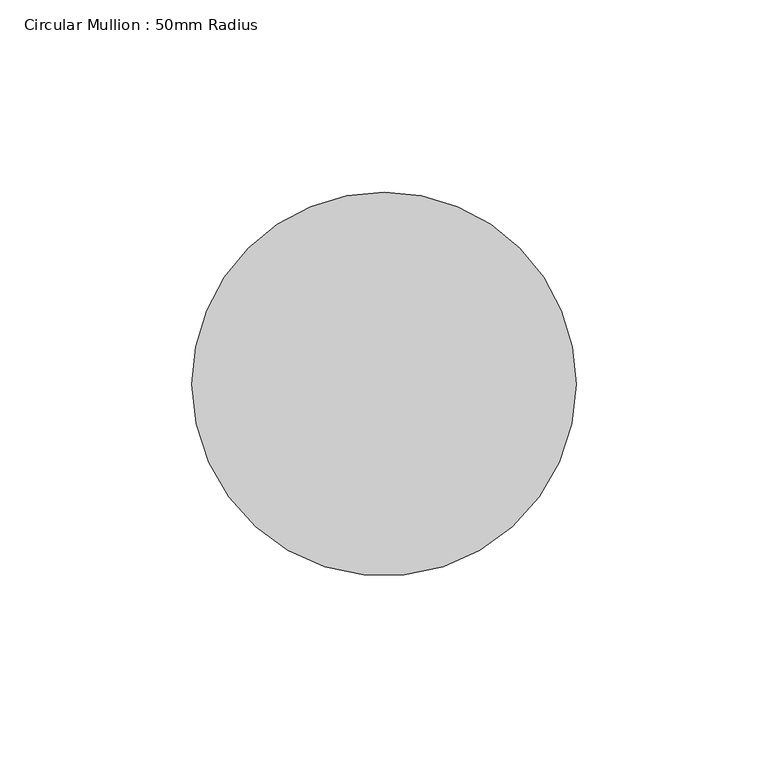
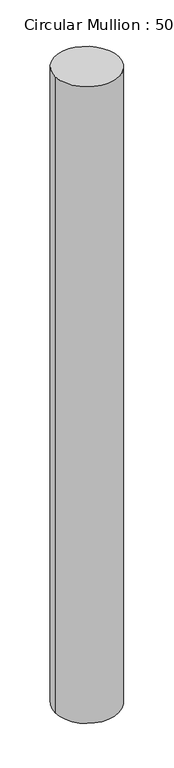
"""IFC4 building model written with IfcOpenShell, lengths in millimetres: member geometry, Circular Mullion : 50mm Radius."""

from ifc_helpers import new_model, si_unit, frame, origin, place, context, project, spatial, ellipse_curve, source, transform, mapped, element, save
from ifc_brep_helpers import plane_surface, cylinder_surface, advanced_brep


def circular_mullion_50mm_radius_b9053822(model_context):
    return source(origin(), model_context, "Body", "AdvancedBrep", [
        advanced_brep(
        [(-100.0, 0.0, 2.0377507), (0.0, 0.0, 0.0), (0.0, 0.0, -1049.5147115), (-100.0, 0.0, -1051.4839752)],
        [
            (0, 1, ellipse_curve(frame((-50.0, 0.0, 1.0188753), z_axis=(-0.020368413714274957, -0.0218488541202306, -0.9995537780912026), x_axis=(-0.6815871331343328, -0.7311270308517654, 0.02987046540653323)), 50.0223211, 50.0)),
            (1, 2),
            (2, 3, ellipse_curve(frame((-50.0, 0.0, -1050.4993433), z_axis=(-0.019684430736599763, -0.021115157107318372, 0.9995832498230997), x_axis=(0.6816072296550739, 0.7311485880509135, 0.02886739810046646)), 50.0208462, 50.0)),
            (3, 0),
            (1, 0, ellipse_curve(frame((-50.0, 0.0, 1.0188753), z_axis=(-0.020368413714274957, -0.0218488541202306, -0.9995537780912026), x_axis=(-0.6815871331343328, -0.7311270308517654, 0.02987046540653323)), 50.0223211, 50.0)),
            (3, 2, ellipse_curve(frame((-50.0, 0.0, -1050.4993433), z_axis=(-0.019684430736599763, -0.021115157107318372, 0.9995832498230997), x_axis=(0.6816072296550739, 0.7311485880509135, 0.02886739810046646)), 50.0208462, 50.0)),
        ],
        [
            cylinder_surface(frame((-50.0, 0.0, 0.0), z_axis=(0.0, 0.0, 1.0), x_axis=(1.0, 0.0, 0.0)), 50.0),
            plane_surface(frame((-222.9470028, 207.8405012, 0.0), z_axis=(0.020368413714274957, 0.0218488541202306, 0.9995537780912026), x_axis=(0.6815871331343322, 0.731127030851766, -0.029870465406534624))),
            plane_surface(frame((-222.9470028, 207.8405012, -1049.5147115), z_axis=(0.019684430736599763, 0.021115157107318372, -0.9995832498230997), x_axis=(0.681607229655074, 0.7311485880509135, 0.028867398100465014))),
        ],
        [
            (0, [[1, 2, 3, 4]]),
            (0, [[5, -4, 6, -2]]),
            (1, [[-1, -5]]),
            (2, [[-6, -3]]),
        ],
    ),
    ])


if __name__ == "__main__":
    model = new_model("IFC4")
    model_context = context("Model", 3, world=origin())
    ifc_project = project(units=[si_unit("LENGTHUNIT", "METRE", prefix="MILLI")], contexts=[model_context])
    site = spatial("IfcSite", under=ifc_project)
    building = spatial("IfcBuilding", under=site)
    placement = place(None, origin())
    circular_mullion_50mm_radius_shape = circular_mullion_50mm_radius_b9053822(model_context)
    element("IfcMember", 1, ObjectType="Circular Mullion : 50mm Radius", at=placement, inside=building, context=model_context, shape_type="MappedRepresentation", body=[
        mapped(circular_mullion_50mm_radius_shape, transform((0.0, 0.0, 0.0), x_axis=(1.0, 0.0, 0.0), y_axis=(0.0, 1.0, 0.0), z_axis=(0.0, 0.0, 1.0))),
    ])
    save(model, "model.ifc")

# Revit data of these elements
# Type "Circular Mullion : 50mm Radius"
#   built-in parameter 1007350 = 0.164042 (stored number, unit not read)
# Element 1 (IfcMember, "Circular Mullion : 50mm Radius")
#   Materials on its faces: "Aluminium"
# Materials
#   "Aluminium": class "Metal", colour RGB 247 247 247, transparency 0, Description = "Aluminium 6061", Cost = 0
